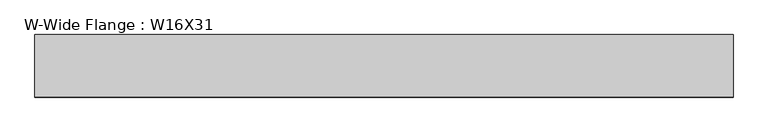
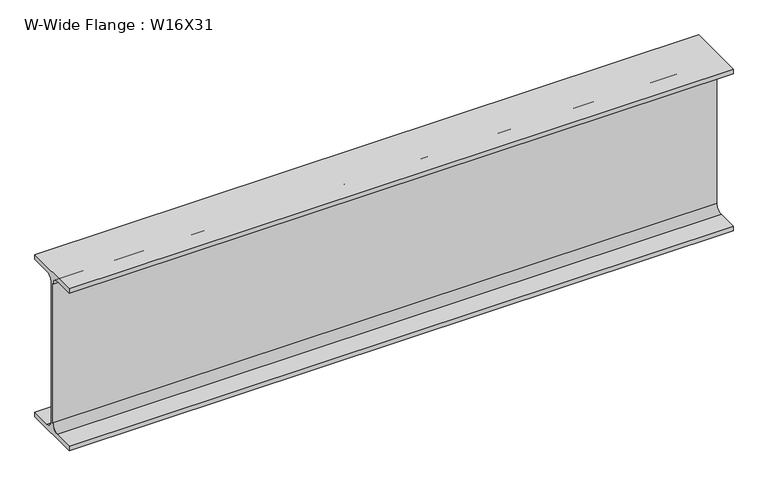
"""IFC4 building model written with IfcOpenShell, lengths in millimetres: beam geometry, W-Wide Flange : W16X31."""

import ifcopenshell
import ifcopenshell.guid

model = None  # the IFC model being written
_history = None  # IfcOwnerHistory: only IFC2X3 demands one
_inside = {}  # id of a spatial element -> (the spatial element, [elements in it])
_under = {}  # id of a project, library or spatial element -> (it, [spatial elements below it])
_declared = {}  # id of a project -> (the project, [libraries it declares])
_typed = {}  # id of a type object -> (the type object, [elements of that type])
_made_of = {}  # id of a material, layer set ... -> (it, [elements and type objects made of it])


def new_model(schema):
    """Start an empty IFC model of exactly this schema.

    Asked for "IFC4X3", IfcOpenShell would pick the latest addendum, in which some entities
    have other attributes; the version numbers below select the first issue.
    IFC2X3 requires an IfcOwnerHistory on every rooted entity: one is made here for all.
    """
    global model, _history
    if schema == "IFC4X3":
        model = ifcopenshell.file(schema_version=(4, 3, 0, 0))
    else:
        model = ifcopenshell.file(schema=schema)
    _inside.clear()
    _under.clear()
    _declared.clear()
    _typed.clear()
    _made_of.clear()
    _history = None
    if model.schema == "IFC2X3":
        org = make("IfcOrganization", Name="unknown")
        user = make(
            "IfcPersonAndOrganization",
            ThePerson=make("IfcPerson", FamilyName="unknown"),
            TheOrganization=org,
        )
        app = make(
            "IfcApplication",
            ApplicationDeveloper=org,
            Version="unknown",
            ApplicationFullName="unknown",
            ApplicationIdentifier="unknown",
        )
        _history = make(
            "IfcOwnerHistory",
            OwningUser=user,
            OwningApplication=app,
            ChangeAction="ADDED",
            CreationDate=0,
        )
    return model


def make(cls, **values):
    """One entity of the class cls with the attributes given. An attribute that is None is left unset."""
    return model.create_entity(
        cls, **{name: value for name, value in values.items() if value is not None}
    )


def rooted(cls, **values):
    """An entity with a GlobalId (a new one), such as an element, a storey or a relation."""
    return make(cls, GlobalId=ifcopenshell.guid.new(), OwnerHistory=_history, **values)


def si_unit(unit_type, name, prefix=None):
    """IfcSIUnit, for example si_unit("LENGTHUNIT", "METRE", prefix="MILLI")."""
    return make("IfcSIUnit", UnitType=unit_type, Prefix=prefix, Name=name)


def assignment(units):
    """IfcUnitAssignment: the units of a project."""
    return None if units is None else make("IfcUnitAssignment", Units=units)


def point(xyz):
    """IfcCartesianPoint."""
    return None if xyz is None else make("IfcCartesianPoint", Coordinates=xyz)


def direction(xyz):
    """IfcDirection."""
    return None if xyz is None else make("IfcDirection", DirectionRatios=xyz)


def frame(location, z_axis=None, x_axis=None):
    """IfcAxis2Placement3D, a coordinate frame: its origin and axes. An axis left out is left unset."""
    return make(
        "IfcAxis2Placement3D",
        Location=point(location),
        Axis=direction(z_axis),
        RefDirection=direction(x_axis),
    )


def frame_2d(location, x_axis=None):
    """IfcAxis2Placement2D, a coordinate frame in the plane: its origin and x axis."""
    return make(
        "IfcAxis2Placement2D", Location=point(location), RefDirection=direction(x_axis)
    )


def origin():
    """The frame at (0, 0, 0) with its axes left unset."""
    return frame((0.0, 0.0, 0.0))


def place(relative_to, where):
    """IfcLocalPlacement: puts the frame where relative to a parent placement (None: the world)."""
    return make(
        "IfcLocalPlacement", PlacementRelTo=relative_to, RelativePlacement=where
    )


def context(
    kind, dimensions, precision=None, world=None, true_north=None, identifier=None
):
    """IfcGeometricRepresentationContext, for example the 3D "Model" context."""
    return make(
        "IfcGeometricRepresentationContext",
        ContextIdentifier=identifier,
        ContextType=kind,
        CoordinateSpaceDimension=dimensions,
        Precision=precision,
        WorldCoordinateSystem=world,
        TrueNorth=true_north,
    )


def project(units=None, contexts=None):
    """IfcProject with its units and contexts."""
    return rooted(
        "IfcProject",
        Name="project",
        RepresentationContexts=contexts,
        UnitsInContext=assignment(units),
    )


def spatial(cls, under=None, at=None, **own):
    """A site, building, storey or space (cls), placed at a placement, below another one or the project."""
    s = rooted(cls, ObjectPlacement=at, **own)
    if under is not None:
        _under.setdefault(under.id(), (under, []))[1].append(s)
    return s


def polyline(points):
    """IfcPolyline through the points."""
    return make("IfcPolyline", Points=[point(p) for p in points])


def circle_curve(where, radius):
    """IfcCircle in the frame where."""
    return make("IfcCircle", Position=where, Radius=radius)


def trimmed(basis, trim1, trim2, sense, master):
    """IfcTrimmedCurve: the piece of a basis curve between two trims."""
    return make(
        "IfcTrimmedCurve",
        BasisCurve=basis,
        Trim1=trim1,
        Trim2=trim2,
        SenseAgreement=sense,
        MasterRepresentation=master,
    )


def segment(curve, same_sense, transition):
    """IfcCompositeCurveSegment."""
    return make(
        "IfcCompositeCurveSegment",
        Transition=transition,
        SameSense=same_sense,
        ParentCurve=curve,
    )


def composite_curve(segments, self_intersect=None):
    """IfcCompositeCurve: segments joined end to end."""
    return make("IfcCompositeCurve", Segments=segments, SelfIntersect=self_intersect)


def outline(outer, holes=None, kind="AREA"):
    """IfcArbitraryClosedProfileDef: a profile drawn as a closed curve; with holes, ...WithVoids."""
    if holes is None:
        return make("IfcArbitraryClosedProfileDef", ProfileType=kind, OuterCurve=outer)
    return make(
        "IfcArbitraryProfileDefWithVoids",
        ProfileType=kind,
        OuterCurve=outer,
        InnerCurves=holes,
    )


def extrude(swept, where, along, depth):
    """IfcExtrudedAreaSolid: the profile swept, set in the frame where, extruded along a direction by depth."""
    return make(
        "IfcExtrudedAreaSolid",
        SweptArea=swept,
        Position=where,
        ExtrudedDirection=direction(along),
        Depth=depth,
    )


def shape(context_of_items, identifier, shape_type, items):
    """IfcShapeRepresentation: the items that make up one representation, for example the "Body"."""
    return make(
        "IfcShapeRepresentation",
        ContextOfItems=context_of_items,
        RepresentationIdentifier=identifier,
        RepresentationType=shape_type,
        Items=items,
    )


def source(mapping_origin, context_of_items, identifier, shape_type, items):
    """IfcRepresentationMap: a shape defined once, which mapped items show again and again."""
    return make(
        "IfcRepresentationMap",
        MappingOrigin=mapping_origin,
        MappedRepresentation=shape(context_of_items, identifier, shape_type, items),
    )


def transform(
    local_origin,
    x_axis=None,
    y_axis=None,
    z_axis=None,
    scale=None,
    scale2=None,
    scale3=None,
    uniform=True,
):
    """IfcCartesianTransformationOperator3D, or its non-uniform kind. x_axis, y_axis, z_axis: its Axis1, 2, 3."""
    if uniform:
        return make(
            "IfcCartesianTransformationOperator3D",
            Axis1=direction(x_axis),
            Axis2=direction(y_axis),
            LocalOrigin=point(local_origin),
            Scale=scale,
            Axis3=direction(z_axis),
        )
    return make(
        "IfcCartesianTransformationOperator3DnonUniform",
        Axis1=direction(x_axis),
        Axis2=direction(y_axis),
        LocalOrigin=point(local_origin),
        Scale=scale,
        Axis3=direction(z_axis),
        Scale2=scale2,
        Scale3=scale3,
    )


def mapped(mapping_source, mapping_target):
    """IfcMappedItem: shows the shape of a source again, moved by a transform."""
    return make(
        "IfcMappedItem", MappingSource=mapping_source, MappingTarget=mapping_target
    )


def made_of(thing, what):
    """Note that an element or type object is made of a material, layer set ...; save() writes the relation."""
    if what is not None:
        _made_of.setdefault(what.id(), (what, []))[1].append(thing)
    return thing


def element(
    cls,
    number,
    at=None,
    inside=None,
    cuts=None,
    type_object=None,
    material=None,
    context=None,
    identifier="Body",
    shape_type=None,
    held_by="IfcProductDefinitionShape",
    body=None,
    shapes=None,
    **own,
):
    """One element of the class cls, such as IfcWall. Its Tag is "e" and its number.

    at: its placement. inside: the storey or other place that contains it. cuts: it is an
    opening in that element (IfcRelVoidsElement). A single representation is given by context,
    identifier, shape_type and body (its items); several are given by shapes. held_by: the class
    of the entity that holds the representations. save() writes the other relations.
    """
    e = rooted(cls, Tag="e%d" % number, ObjectPlacement=at, **own)
    if body is not None:
        shapes = [shape(context, identifier, shape_type, body)]
    if shapes is not None:
        e.Representation = make(held_by, Representations=shapes)
    if inside is not None:
        _inside.setdefault(inside.id(), (inside, []))[1].append(e)
    if cuts is not None:
        rooted(
            "IfcRelVoidsElement", RelatingBuildingElement=cuts, RelatedOpeningElement=e
        )
    if type_object is not None:
        _typed.setdefault(type_object.id(), (type_object, []))[1].append(e)
    return made_of(e, material)


def aggregate(whole, parts):
    """IfcRelAggregates: a whole, such as a stair, and the parts it consists of."""
    return rooted("IfcRelAggregates", RelatingObject=whole, RelatedObjects=parts)


def save(model, path):
    """Write the relations noted so far, then the file.

    IfcRelAggregates (storeys below a building ...), IfcRelContainedInSpatialStructure (elements
    in a storey), IfcRelDefinesByType, IfcRelAssociatesMaterial and IfcRelDeclares: one each for
    every whole, place, type object, material and project.
    """
    for whole, parts in _under.values():
        aggregate(whole, parts)
    for where, things in _inside.values():
        rooted(
            "IfcRelContainedInSpatialStructure",
            RelatedElements=things,
            RelatingStructure=where,
        )
    for kind, things in _typed.values():
        rooted("IfcRelDefinesByType", RelatedObjects=things, RelatingType=kind)
    for what, things in _made_of.values():
        rooted("IfcRelAssociatesMaterial", RelatedObjects=things, RelatingMaterial=what)
    for by, libraries in _declared.values():
        rooted("IfcRelDeclares", RelatingContext=by, RelatedDefinitions=libraries)
    model.write(path)


def w_wide_flange_w16x31_dc2757f3(model_context):
    return source(origin(), model_context, "Body", "SweptSolid", [
        extrude(outline(composite_curve([segment(polyline([(70.231, -190.754), (70.231, -201.93), (-70.231, -201.93), (-70.231, -190.754), (-20.8915, -190.754)]), True, "CONTINUOUS"), segment(trimmed(circle_curve(frame_2d((-20.8915, -173.355)), 17.399), [point((-20.8915, -190.754))], [point((-3.4925, -173.355))], True, "CARTESIAN"), True, "CONTINUOUS"), segment(polyline([(-3.4925, -173.355), (-3.4925, 173.355)]), True, "CONTINUOUS"), segment(trimmed(circle_curve(frame_2d((-20.8915, 173.355)), 17.399), [point((-3.4925, 173.355))], [point((-20.8915, 190.754))], True, "CARTESIAN"), True, "CONTINUOUS"), segment(polyline([(-20.8915, 190.754), (-70.231, 190.754), (-70.231, 201.93), (70.231, 201.93), (70.231, 190.754), (20.8915, 190.754)]), True, "CONTINUOUS"), segment(trimmed(circle_curve(frame_2d((20.8915, 173.355)), 17.399), [point((20.8915, 190.754))], [point((3.4925, 173.355))], True, "CARTESIAN"), True, "CONTINUOUS"), segment(polyline([(3.4925, 173.355), (3.4925, -173.355)]), True, "CONTINUOUS"), segment(trimmed(circle_curve(frame_2d((20.8915, -173.355)), 17.399), [point((3.4925, -173.355))], [point((20.8915, -190.754))], True, "CARTESIAN"), True, "CONTINUOUS"), segment(polyline([(20.8915, -190.754), (70.231, -190.754)]), True, "CONTINUOUS")], self_intersect=False)), frame((-768.7703128, 0.0, 0.0), z_axis=(1.0, 0.0, 0.0), x_axis=(0.0, 1.0, 0.0)), (0.0, 0.0, 1.0), 1567.4788026),
    ])


if __name__ == "__main__":
    model = new_model("IFC4")
    model_context = context("Model", 3, world=origin())
    ifc_project = project(units=[si_unit("LENGTHUNIT", "METRE", prefix="MILLI")], contexts=[model_context])
    site = spatial("IfcSite", under=ifc_project)
    building = spatial("IfcBuilding", under=site)
    placement = place(None, origin())
    w_wide_flange_w16x31_shape = w_wide_flange_w16x31_dc2757f3(model_context)
    element("IfcBeam", 1, ObjectType="W-Wide Flange : W16X31", at=placement, inside=building, context=model_context, shape_type="MappedRepresentation", body=[
        mapped(w_wide_flange_w16x31_shape, transform((0.0, 0.0, 0.0), x_axis=(1.0, 0.0, 0.0), y_axis=(0.0, 1.0, 0.0), z_axis=(0.0, 0.0, 1.0))),
    ])
    save(model, "model.ifc")

# Revit data of these elements
# Type "W-Wide Flange : W16X31"
#   Assembly Code = "B10"
#   W = 31
#   Start Extension Calculation [instance default] = 10' - 0"
#   Start Extension [instance default] = -0' - 0 1/2"
#   End Extension Calculation [instance default] = 10' - 0"
#   End Extension [instance default] = -0' - 0 1/2"
#   Length [instance default] = 5' - 0"
#   bf = 0' - 5.53"
#   d = 1' - 3.9"
#   k = 0' - 1 1/8"
#   k2 = 0' - 0.685"
#   tf = 0' - 0.44"
#   tw = 0' - 0.275"
#   A = 0.0634028 SF
#   Beam Material [instance default] = Metal - Steel - ASTM A992
# Element 1 (IfcBeam, "W-Wide Flange : W16X31")
#   Materials on its faces: "Metal - Steel - ASTM A992"
# Materials
#   "Metal - Steel - ASTM A992": class "Metal", colour RGB 128 0 0, transparency 0
